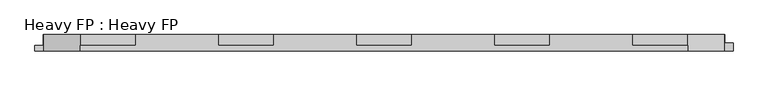
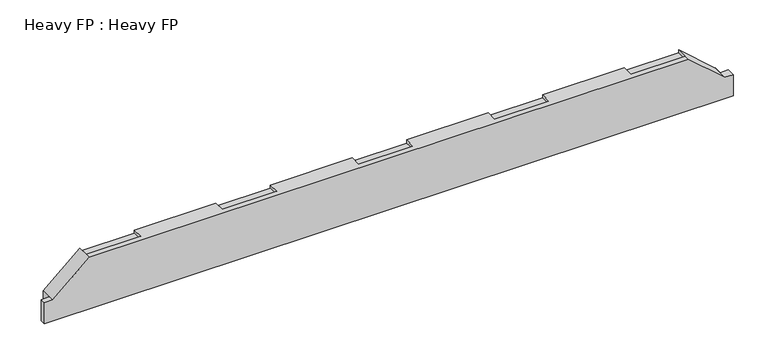
"""IFC4 building model written with IfcOpenShell, lengths in millimetres: beam geometry, Heavy FP : Heavy FP."""

from ifc_helpers import new_model, si_unit, origin, place, context, project, spatial, faceted_brep, source, transform, mapped, element, save


def heavy_fp_heavy_fp_30e82a3a(model_context):
    return source(origin(), model_context, "Body", "Brep", [
        faceted_brep([(50483.2245514, 50679.9999991, 13800.0), (50483.2245514, 50679.9999991, 14620.0), (50170.5245515, 50679.9999991, 14620.0), (48833.2245515, 50679.9999991, 15800.0), (26833.2245515, 50679.9999991, 15800.0), (25495.9245515, 50679.9999991, 14620.0), (25183.2245519, 50679.9999991, 14620.0), (25183.2245519, 50679.9999991, 13800.0), (25495.9245515, 51279.9999991, 14620.0), (26833.2245515, 51279.9999991, 15800.0), (26833.2245515, 51279.9999991, 15680.0), (28833.2245515, 51279.9999991, 15680.0), (28833.2245515, 51279.9999991, 15800.0), (31833.2245515, 51279.9999991, 15800.0), (31833.2245515, 51279.9999991, 15680.0), (33833.2245515, 51279.9999991, 15680.0), (33833.2245515, 51279.9999991, 15800.0), (36833.2245515, 51279.9999991, 15800.0), (36833.2245515, 51279.9999991, 15680.0), (38833.2245515, 51279.9999991, 15680.0), (38833.2245515, 51279.9999991, 15800.0), (41833.2245515, 51279.9999991, 15800.0), (41833.2245515, 51279.9999991, 15680.0), (43833.2245515, 51279.9999991, 15680.0), (43833.2245515, 51279.9999991, 15800.0), (46833.2245515, 51279.9999991, 15800.0), (46833.2245515, 51279.9999991, 15680.0), (48833.2245515, 51279.9999991, 15680.0), (48833.2245515, 51279.9999991, 15800.0), (50170.5245515, 51279.9999991, 14620.0), (50183.2245514, 51279.9999991, 14620.0), (50183.2245514, 51279.9999991, 13800.0), (45483.2245512, 51279.9999991, 13800.0), (45483.2245512, 51279.9999991, 14620.0), (45183.2245512, 51279.9999991, 14620.0), (45183.2245512, 51279.9999991, 13800.0), (40483.2245513, 51279.9999991, 13800.0), (40483.2245513, 51279.9999991, 14620.0), (40183.2245513, 51279.9999991, 14620.0), (40183.2245513, 51279.9999991, 13800.0), (35483.2245514, 51279.9999991, 13800.0), (35483.2245514, 51279.9999991, 14620.0), (35183.2245514, 51279.9999991, 14620.0), (35183.2245514, 51279.9999991, 13800.0), (30483.2245515, 51279.9999991, 13800.0), (30483.2245515, 51279.9999991, 14620.0), (30183.2245515, 51279.9999991, 14620.0), (30183.2245515, 51279.9999991, 13800.0), (25483.2245516, 51279.9999991, 13800.0), (25483.2245516, 51279.9999991, 14620.0), (50483.2245514, 50979.9999988, 13800.0), (50483.2245514, 50979.9999988, 14620.0), (50183.2245514, 50979.9999988, 14620.0), (48833.2245515, 50879.7448203, 15800.0), (46833.2245515, 50879.7448203, 15800.0), (43833.2245515, 50879.7448203, 15800.0), (41833.2245515, 50879.7448203, 15800.0), (38833.2245515, 50879.7448203, 15800.0), (36833.2245515, 50879.7448203, 15800.0), (33833.2245515, 50879.7448203, 15800.0), (31833.2245515, 50879.7448203, 15800.0), (28833.2245515, 50879.7448203, 15800.0), (26833.2245515, 50879.7448203, 15800.0), (25483.2245516, 50879.7448219, 14620.0), (25183.2245519, 50879.7448219, 14620.0), (25183.2245519, 50879.7448219, 13800.0), (25483.2245516, 50879.7448219, 13800.0), (30183.2245515, 50979.9999991, 13800.0), (30483.2245515, 50979.9999991, 13800.0), (35183.2245514, 50979.9999991, 13800.0), (35483.2245514, 50979.9999991, 13800.0), (40183.2245513, 50979.9999991, 13800.0), (40483.2245513, 50979.9999991, 13800.0), (45183.2245512, 50979.9999991, 13800.0), (45483.2245512, 50979.9999991, 13800.0), (50183.2245514, 50979.9999988, 13800.0), (30183.2245515, 50979.9999991, 14620.0), (30483.2245515, 50979.9999991, 14620.0), (35183.2245514, 50979.9999991, 14620.0), (35483.2245514, 50979.9999991, 14620.0), (40183.2245513, 50979.9999991, 14620.0), (40483.2245513, 50979.9999991, 14620.0), (45183.2245512, 50979.9999991, 14620.0), (45483.2245512, 50979.9999991, 14620.0), (46833.2245515, 50879.7448203, 15680.0), (48833.2245515, 50879.7448203, 15680.0), (41833.2245515, 50879.7448203, 15680.0), (43833.2245515, 50879.7448203, 15680.0), (36833.2245515, 50879.7448203, 15680.0), (38833.2245515, 50879.7448203, 15680.0), (31833.2245515, 50879.7448203, 15680.0), (33833.2245515, 50879.7448203, 15680.0), (26833.2245515, 50879.7448203, 15680.0), (28833.2245515, 50879.7448203, 15680.0)], [[[0, 1, 2, 3, 4, 5, 6, 7]], [[8, 9, 10, 11, 12, 13, 14, 15, 16, 17, 18, 19, 20, 21, 22, 23, 24, 25, 26, 27, 28, 29, 30, 31, 32, 33, 34, 35, 36, 37, 38, 39, 40, 41, 42, 43, 44, 45, 46, 47, 48, 49]], [[1, 0, 50, 51]], [[2, 1, 51, 52, 30, 29]], [[3, 2, 29, 28, 53]], [[4, 3, 53, 54, 25, 24, 55, 56, 21, 20, 57, 58, 17, 16, 59, 60, 13, 12, 61, 62]], [[5, 4, 62, 9, 8]], [[6, 5, 8, 49, 63, 64]], [[7, 6, 64, 65]], [[0, 7, 65, 66, 48, 47, 67, 68, 44, 43, 69, 70, 40, 39, 71, 72, 36, 35, 73, 74, 32, 31, 75, 50]], [[67, 76, 77, 68]], [[77, 76, 46, 45]], [[68, 77, 45, 44]], [[76, 67, 47, 46]], [[69, 78, 79, 70]], [[79, 78, 42, 41]], [[70, 79, 41, 40]], [[78, 69, 43, 42]], [[71, 80, 81, 72]], [[81, 80, 38, 37]], [[72, 81, 37, 36]], [[80, 71, 39, 38]], [[73, 82, 83, 74]], [[83, 82, 34, 33]], [[74, 83, 33, 32]], [[82, 73, 35, 34]], [[84, 85, 27, 26]], [[85, 53, 28, 27]], [[85, 84, 54, 53]], [[54, 84, 26, 25]], [[86, 87, 23, 22]], [[87, 55, 24, 23]], [[87, 86, 56, 55]], [[56, 86, 22, 21]], [[88, 89, 19, 18]], [[89, 57, 20, 19]], [[89, 88, 58, 57]], [[58, 88, 18, 17]], [[90, 91, 15, 14]], [[91, 59, 16, 15]], [[91, 90, 60, 59]], [[60, 90, 14, 13]], [[92, 93, 11, 10]], [[93, 61, 12, 11]], [[93, 92, 62, 61]], [[62, 92, 10, 9]], [[66, 63, 49, 48]], [[63, 66, 65, 64]], [[52, 75, 31, 30]], [[75, 52, 51, 50]]]),
    ])


if __name__ == "__main__":
    model = new_model("IFC4")
    model_context = context("Model", 3, world=origin())
    ifc_project = project(units=[si_unit("LENGTHUNIT", "METRE", prefix="MILLI")], contexts=[model_context])
    site = spatial("IfcSite", under=ifc_project)
    building = spatial("IfcBuilding", under=site)
    placement = place(None, origin())
    heavy_fp_heavy_fp_shape = heavy_fp_heavy_fp_30e82a3a(model_context)
    element("IfcBeam", 1, ObjectType="Heavy FP : Heavy FP", at=placement, inside=building, context=model_context, shape_type="MappedRepresentation", body=[
        mapped(heavy_fp_heavy_fp_shape, transform((0.0, 0.0, 0.0), x_axis=(1.0, 0.0, 0.0), y_axis=(0.0, 1.0, 0.0), z_axis=(0.0, 0.0, 1.0))),
    ])
    save(model, "model.ifc")
